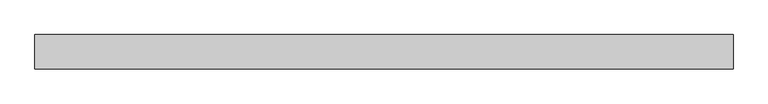
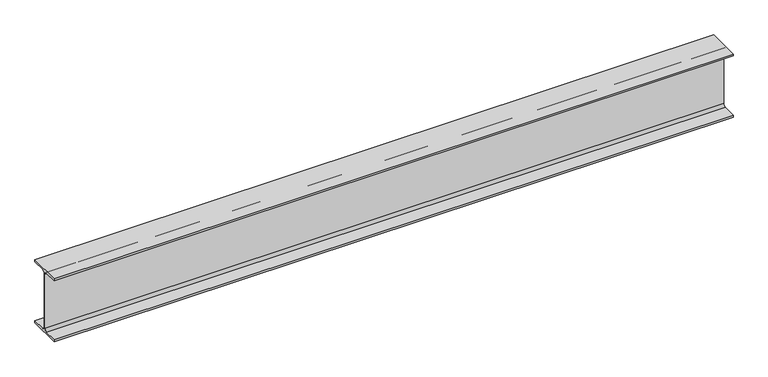
"""IFC4 building model written with IfcOpenShell, lengths in millimetres: beam geometry, 0912_Steel Framing_H-KSD3502 : H_SB_AR_S02_H-350x175x7x11_Platform."""

from ifc_helpers import new_model, si_unit, point, frame, frame_2d, origin, place, context, project, spatial, polyline, circle_curve, trimmed, segment, composite_curve, outline, extrude, source, transform, mapped, element, save


def beam_9c24ba7d(model_context):
    return source(origin(), model_context, "Body", "SweptSolid", [
        extrude(outline(composite_curve([segment(polyline([(87.5, -164.0), (87.5, -175.0), (-87.5, -175.0), (-87.5, -164.0), (-17.5, -164.0)]), True, "CONTINUOUS"), segment(trimmed(circle_curve(frame_2d((-17.5, -150.0)), 14.0), [point((-17.5, -164.0))], [point((-3.5, -150.0))], True, "CARTESIAN"), True, "CONTINUOUS"), segment(polyline([(-3.5, -150.0), (-3.5, 150.0)]), True, "CONTINUOUS"), segment(trimmed(circle_curve(frame_2d((-17.5, 150.0)), 14.0), [point((-3.5, 150.0))], [point((-17.5, 164.0))], True, "CARTESIAN"), True, "CONTINUOUS"), segment(polyline([(-17.5, 164.0), (-87.5, 164.0), (-87.5, 175.0), (87.5, 175.0), (87.5, 164.0), (17.5, 164.0)]), True, "CONTINUOUS"), segment(trimmed(circle_curve(frame_2d((17.5, 150.0)), 14.0), [point((17.5, 164.0))], [point((3.5, 150.0))], True, "CARTESIAN"), True, "CONTINUOUS"), segment(polyline([(3.5, 150.0), (3.5, -150.0)]), True, "CONTINUOUS"), segment(trimmed(circle_curve(frame_2d((17.5, -150.0)), 14.0), [point((3.5, -150.0))], [point((17.5, -164.0))], True, "CARTESIAN"), True, "CONTINUOUS"), segment(polyline([(17.5, -164.0), (87.5, -164.0)]), True, "CONTINUOUS")], self_intersect=False)), frame((-1811.887571, 0.0, 0.0), z_axis=(1.0, 0.0, 0.0), x_axis=(0.0, 1.0, 0.0)), (0.0, 0.0, 1.0), 3566.8249285),
    ])


if __name__ == "__main__":
    model = new_model("IFC4")
    model_context = context("Model", 3, world=origin())
    ifc_project = project(units=[si_unit("LENGTHUNIT", "METRE", prefix="MILLI")], contexts=[model_context])
    site = spatial("IfcSite", under=ifc_project)
    building = spatial("IfcBuilding", under=site)
    placement = place(None, origin())
    beam_shape = beam_9c24ba7d(model_context)
    element("IfcBeam", 1, ObjectType="0912_Steel Framing_H-KSD3502 : H_SB_AR_S02_H-350x175x7x11_Platform", at=placement, inside=building, context=model_context, shape_type="MappedRepresentation", body=[
        mapped(beam_shape, transform((0.0, 0.0, 0.0), x_axis=(1.0, 0.0, 0.0), y_axis=(0.0, 1.0, 0.0), z_axis=(0.0, 0.0, 1.0))),
    ])
    save(model, "model.ifc")

# Revit data of these elements
# Type "0912_Steel Framing_H-KSD3502 : H_SB_AR_S02_H-350x175x7x11_Platform"
#   H_Q'ty Cal Type Tag = "SB-Q2"
#   H_WM Code_1 = "S01AA073-00001 |  | TON | Main Steel Structure Fabrication Work | Shelter/Building | Medium Steel - Standard |  |  |  |  |  |  | Material: (   ) | (90)KG/M>Weight≥(30)KG/M | S01AA073-00001 Main Steel Structure Fabrication Work Shelter/Building Medium Steel - Standard         | - Material: ( ASTM A36 )\n- (90)KG/M>Weight≥(30)KG/M"
#   H_WM Code_2 = "S03AA083-00001 |  | TON | Main Steel Structure Erection Work | Shelter/Building | Medium Steel |  |  |  |  |  |  | Material: (   ) | S03AA083-00001 Main Steel Structure Erection Work Shelter/Building Medium Steel         | - Material: ( ASTM A36 )"
#   H_WM Code_3 = "S01AA009-00001 |  | TON | Main Steel Structure Fabrication Work | Shelter/Building | Plates - Gusset, Stiffener, ETC | Material: (   ) | S01AA009-00001 Main Steel Structure Fabrication Work Shelter/Building Plates - Gusset, Stiffener, ETC         |"
#   H_WM Code_4 = "S41AA051-00001 |  | M2 | Steel Structure Paint Work | Shelter/Building | for Non-Fireproofed Steel Surface |  |  |  |  |  |  | Material: (   ) | S41AA051-00001 Steel Structure Paint Work Shelter/Building for Non-Fireproofed Steel Surface         |"
#   Width = 17.5 cm
#   Web Thickness = 0.7 cm
#   Web Fillet = 1.4 cm
#   Warping Constant = 282000.0 cm⁶
#   W = 0
#   Torsional Moment of Inertia = 19.4042 cm⁴
#   Section Area = 63.14 cm²
#   Plastic Modulus weak axis = 174.0 cm³
#   Plastic Modulus strong axis = 868.0 cm³
#   Perimeter = 1.36 m²/m
#   Nominal Weight = 49.60 kgf/m
#   Moment of Inertia weak axis = 984.00 cm⁴
#   Moment of Inertia strong axis = 13600.00 cm⁴
#   Height = 35.0 cm
#   Flange Thickness = 1.1 cm
#   Elastic Modulus weak axis = 112.0 cm³
#   Elastic Modulus strong axis = 775.0 cm³
#   Centroid Vertical = 17.5 cm
#   Centroid Horizontal = 8.75 cm
#   Ix = 136000000
#   Length [instance default] = 1524 mm
#   Zx = 868000
#   b = 175 mm
#   h = 350 mm
#   r = 14 mm
#   s = 7 mm
#   t = 11 mm
#   A = 0.006314 m²
#   Structural Material [instance default] = Steel, 45-345
#   Assembly Code = ""
# Element 1 (IfcBeam, "0912_Steel Framing_H-KSD3502 : H_SB_AR_S02_H-350x175x7x11_Platform")
#   Materials on its faces: "Steel, 45-345"
# Materials
#   "Steel, 45-345": class "Metal", colour RGB 189 187 185, transparency 0, Description = "Steel 345 MPa", Cost = 0
